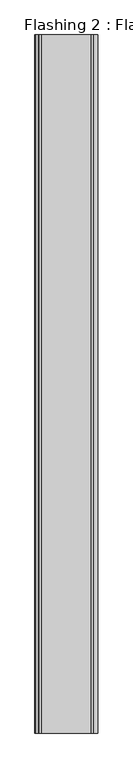
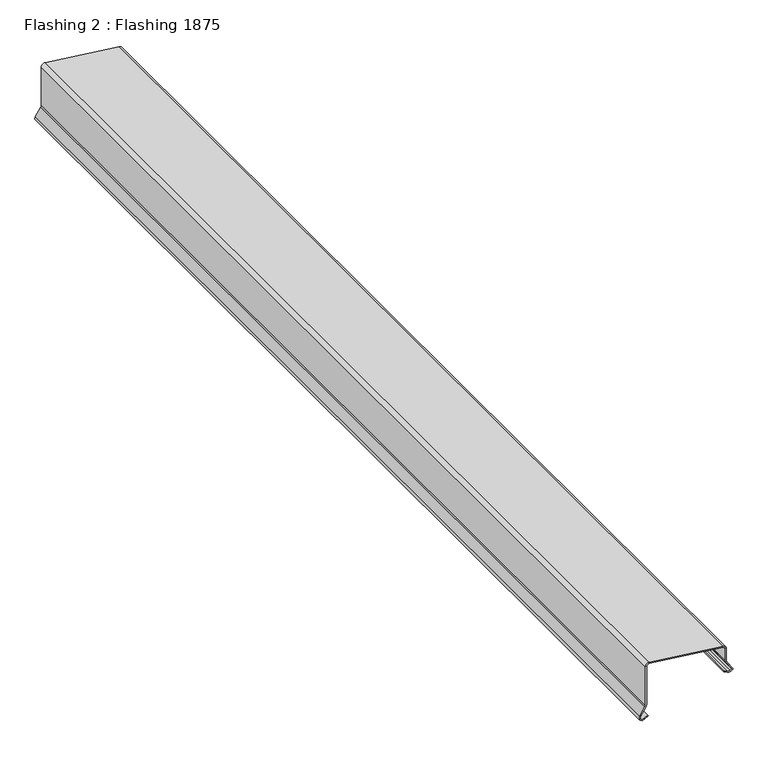
"""IFC4 building model written with IfcOpenShell, lengths in millimetres: proxy geometry, Flashing 2 : Flashing 1875."""

from ifc_helpers import new_model, si_unit, point, frame, frame_2d, origin, place, context, project, spatial, polyline, circle_curve, trimmed, segment, composite_curve, outline, extrude, source, transform, mapped, element, save


def flashing_2_flashing_1875_d6e76b17(model_context):
    return source(origin(), model_context, "Body", "SweptSolid", [
        extrude(outline(composite_curve([segment(trimmed(circle_curve(frame_2d((40133.2517994, -9767.0036771)), 6.35), [point((40127.5360053, -9769.7699376))], [point((40127.867313, -9763.6376994))], False, "CARTESIAN"), True, "CONTINUOUS"), segment(polyline([(40127.867313, -9763.6376994), (40130.8867187, -9758.8076172), (40149.4789842, -9770.8014653)]), True, "CONTINUOUS"), segment(trimmed(circle_curve(frame_2d((40152.9212544, -9765.4654297)), 6.35), [point((40149.4789842, -9770.8014653))], [point((40152.9212544, -9771.8154297))], True, "CARTESIAN"), True, "CONTINUOUS"), segment(polyline([(40152.9212544, -9771.8154297), (40176.1640916, -9771.8154297)]), True, "CONTINUOUS"), segment(trimmed(circle_curve(frame_2d((40176.1640916, -9778.1654297)), 6.35), [point((40176.1640916, -9771.8154297))], [point((40182.4677067, -9777.3993118))], False, "CARTESIAN"), True, "CONTINUOUS"), segment(polyline([(40182.4677067, -9777.3993118), (40199.6976336, -9919.1670852)]), True, "CONTINUOUS"), segment(trimmed(circle_curve(frame_2d((40193.3940184, -9919.9332031)), 6.35), [point((40199.6976336, -9919.1670852))], [point((40193.3940184, -9926.2832031))], False, "CARTESIAN"), True, "CONTINUOUS"), segment(polyline([(40193.3940184, -9926.2832031), (40116.1659228, -9926.2832031)]), True, "CONTINUOUS"), segment(trimmed(circle_curve(frame_2d((40116.1659228, -9932.6332031)), 6.35), [point((40116.1659228, -9926.2832031))], [point((40112.7319037, -9927.2918538))], True, "CARTESIAN"), True, "CONTINUOUS"), segment(polyline([(40112.7319037, -9927.2918538), (40096.8914441, -9937.4758802)]), True, "CONTINUOUS"), segment(trimmed(circle_curve(frame_2d((40093.4574249, -9932.1345309)), 6.35), [point((40096.8914441, -9937.4758802))], [point((40088.1090015, -9935.5575219))], False, "CARTESIAN"), True, "CONTINUOUS"), segment(polyline([(40088.1090015, -9935.5575219), (40086.3359375, -9932.7871094), (40092.1875, -9921.0800781), (40093.9764738, -9921.9742665), (40088.63264, -9932.6655014), (40089.7935443, -9934.4794145)]), True, "CONTINUOUS"), segment(trimmed(circle_curve(frame_2d((40093.4574249, -9932.1345309)), 4.35), [point((40089.7935443, -9934.4794145))], [point((40095.8098632, -9935.7935655))], True, "CARTESIAN"), True, "CONTINUOUS"), segment(polyline([(40095.8098632, -9935.7935655), (40111.6503228, -9925.6095391)]), True, "CONTINUOUS"), segment(trimmed(circle_curve(frame_2d((40116.1659228, -9932.6332031)), 8.35), [point((40111.6503228, -9925.6095391))], [point((40116.1659228, -9924.2832031))], False, "CARTESIAN"), True, "CONTINUOUS"), segment(polyline([(40116.1659228, -9924.2832031), (40193.3940184, -9924.2832031)]), True, "CONTINUOUS"), segment(trimmed(circle_curve(frame_2d((40193.3940184, -9919.9332031)), 4.35), [point((40193.3940184, -9924.2832031))], [point((40197.712243, -9919.4083822))], True, "CARTESIAN"), True, "CONTINUOUS"), segment(polyline([(40197.712243, -9919.4083822), (40180.4823161, -9777.6406088)]), True, "CONTINUOUS"), segment(trimmed(circle_curve(frame_2d((40176.1640916, -9778.1654297)), 4.35), [point((40180.4823161, -9777.6406088))], [point((40176.1640916, -9773.8154297))], True, "CARTESIAN"), True, "CONTINUOUS"), segment(polyline([(40176.1640916, -9773.8154297), (40152.9212544, -9773.8154297)]), True, "CONTINUOUS"), segment(trimmed(circle_curve(frame_2d((40152.9212544, -9765.4654297)), 8.35), [point((40152.9212544, -9773.8154297))], [point((40148.3948046, -9772.4821064))], False, "CARTESIAN"), True, "CONTINUOUS"), segment(polyline([(40148.3948046, -9772.4821064), (40131.5072723, -9761.5879796), (40129.5632143, -9764.6978498)]), True, "CONTINUOUS"), segment(trimmed(circle_curve(frame_2d((40133.2517994, -9767.0036771)), 4.35), [point((40129.5632143, -9764.6978498))], [point((40129.3362554, -9768.8986745))], True, "CARTESIAN"), True, "CONTINUOUS"), segment(polyline([(40129.3362554, -9768.8986745), (40132.6869689, -9775.8220962), (40130.8867187, -9776.6933594), (40127.5360053, -9769.7699376)]), True, "CONTINUOUS")], self_intersect=False)), frame((0.0, 7982.1531721, 0.0), z_axis=(0.0, 1.0, 0.0), x_axis=(0.0, 0.0, 1.0)), (0.0, 0.0, 1.0), 2000.0),
    ])


if __name__ == "__main__":
    model = new_model("IFC4")
    model_context = context("Model", 3, world=origin())
    ifc_project = project(units=[si_unit("LENGTHUNIT", "METRE", prefix="MILLI")], contexts=[model_context])
    site = spatial("IfcSite", under=ifc_project)
    building = spatial("IfcBuilding", under=site)
    placement = place(None, origin())
    flashing_2_flashing_1875_shape = flashing_2_flashing_1875_d6e76b17(model_context)
    element("IfcBuildingElementProxy", 1, Name="Flashing 2 : Flashing 1875", ObjectType="Flashing 2 : Flashing 1875", at=placement, inside=building, context=model_context, shape_type="MappedRepresentation", body=[
        mapped(flashing_2_flashing_1875_shape, transform((0.0, 0.0, 0.0), x_axis=(1.0, 0.0, 0.0), y_axis=(0.0, 1.0, 0.0), z_axis=(0.0, 0.0, 1.0))),
    ])
    save(model, "model.ifc")

# Revit data of these elements
# Type "Flashing 2 : Flashing 1875"
#   NameOverride = "Flashing"
# Element 1 (IfcBuildingElementProxy, "Flashing 2 : Flashing 1875")
#   Materials on its faces: "METAL COPING"
# Materials
#   "METAL COPING": class "Unassigned", colour RGB 128 128 128, transparency 0
